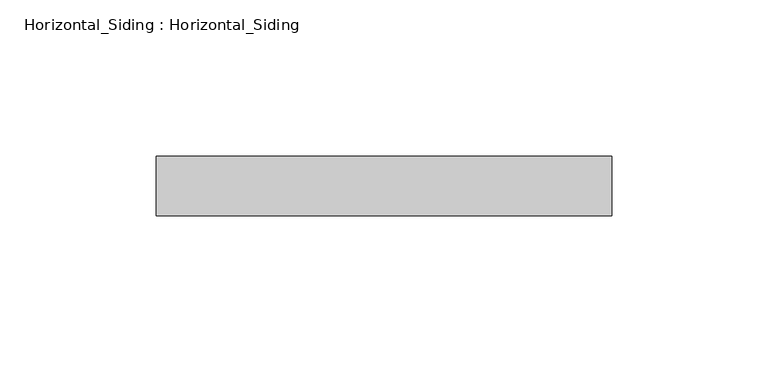
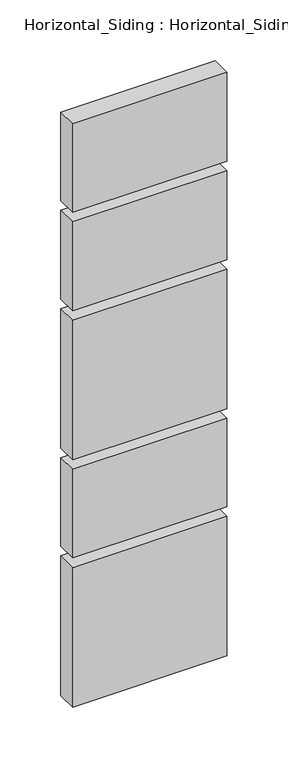
"""IFC4 building model written with IfcOpenShell, lengths in millimetres: plate geometry, Horizontal_Siding : Horizontal_Siding."""

from ifc_helpers import new_model, si_unit, frame, origin, place, context, project, spatial, polyline, outline, extrude, source, transform, mapped, element, save


def horizontal_siding_horizontal_siding_1445cc47(model_context):
    return source(origin(), model_context, "Body", "SweptSolid", [
        extrude(outline(polyline([(73.025, -19.05), (-73.025, -19.05), (-73.025, 0.0), (73.025, 0.0), (73.025, -19.05)])), frame((0.0, 0.0, 9.525), z_axis=(0.0, 0.0, 1.0), x_axis=(1.0, 0.0, 0.0)), (0.0, 0.0, 1.0), 139.7),
        extrude(outline(polyline([(73.025, -19.05), (-73.025, -19.05), (-73.025, 0.0), (73.025, 0.0), (73.025, -19.05)])), frame((0.0, 0.0, 158.75), z_axis=(0.0, 0.0, 1.0), x_axis=(1.0, 0.0, 0.0)), (0.0, 0.0, 1.0), 88.9),
        extrude(outline(polyline([(73.025, -19.05), (-73.025, -19.05), (-73.025, 0.0), (73.025, 0.0), (73.025, -19.05)])), frame((0.0, 0.0, 257.175), z_axis=(0.0, 0.0, 1.0), x_axis=(1.0, 0.0, 0.0)), (0.0, 0.0, 1.0), 139.7),
        extrude(outline(polyline([(73.025, -19.05), (-73.025, -19.05), (-73.025, 0.0), (73.025, 0.0), (73.025, -19.05)])), frame((0.0, 0.0, 406.4), z_axis=(0.0, 0.0, 1.0), x_axis=(1.0, 0.0, 0.0)), (0.0, 0.0, 1.0), 88.9),
        extrude(outline(polyline([(73.025, -19.05), (-73.025, -19.05), (-73.025, 0.0), (73.025, 0.0), (73.025, -19.05)])), frame((0.0, 0.0, 504.825), z_axis=(0.0, 0.0, 1.0), x_axis=(1.0, 0.0, 0.0)), (0.0, 0.0, 1.0), 88.9),
    ])


if __name__ == "__main__":
    model = new_model("IFC4")
    model_context = context("Model", 3, world=origin())
    ifc_project = project(units=[si_unit("LENGTHUNIT", "METRE", prefix="MILLI")], contexts=[model_context])
    site = spatial("IfcSite", under=ifc_project)
    building = spatial("IfcBuilding", under=site)
    placement = place(None, origin())
    horizontal_siding_horizontal_siding_shape = horizontal_siding_horizontal_siding_1445cc47(model_context)
    element("IfcPlate", 1, ObjectType="Horizontal_Siding : Horizontal_Siding", at=placement, inside=building, context=model_context, shape_type="MappedRepresentation", body=[
        mapped(horizontal_siding_horizontal_siding_shape, transform((0.0, 0.0, 0.0), x_axis=(1.0, 0.0, 0.0), y_axis=(0.0, 1.0, 0.0), z_axis=(0.0, 0.0, 1.0))),
    ])
    save(model, "model.ifc")

# Revit data of these elements
# Type "Horizontal_Siding : Horizontal_Siding"
#   Analytic Construction = "<None>"
#   extend = 0' - 2 3/4"
#   Width_2 = 0' - 3 1/2"
#   Width_1 = 0' - 5 1/2"
#   Gap = 0' - 0 3/8"
#   Plank Material = SLOTTED WOOD FENCE (THERMALLY MODIFIED WOOD: ARBOR WOOD)\n(EXTERIOR STAIN : PENOFIN VERDE EXT. STAIN - COLOR: CEDAR)
# Element 1 (IfcPlate, "Horizontal_Siding : Horizontal_Siding")
#   Materials on its faces: "SLOTTED WOOD FENCE (THERMALLY MODIFIED WOOD: ARBOR WOOD)\n(EXTERIOR STAIN : PENOFIN VERDE EXT. STAIN - COLOR: CEDAR)"
# Materials
#   "SLOTTED WOOD FENCE (THERMALLY MODIFIED WOOD: ARBOR WOOD)\n(EXTERIOR STAIN : PENOFIN VERDE EXT. STAIN - COLOR: CEDAR)": class "Wood", colour RGB 164 134 123, transparency 0, Description = "Pinus Echinata", Cost = 0
